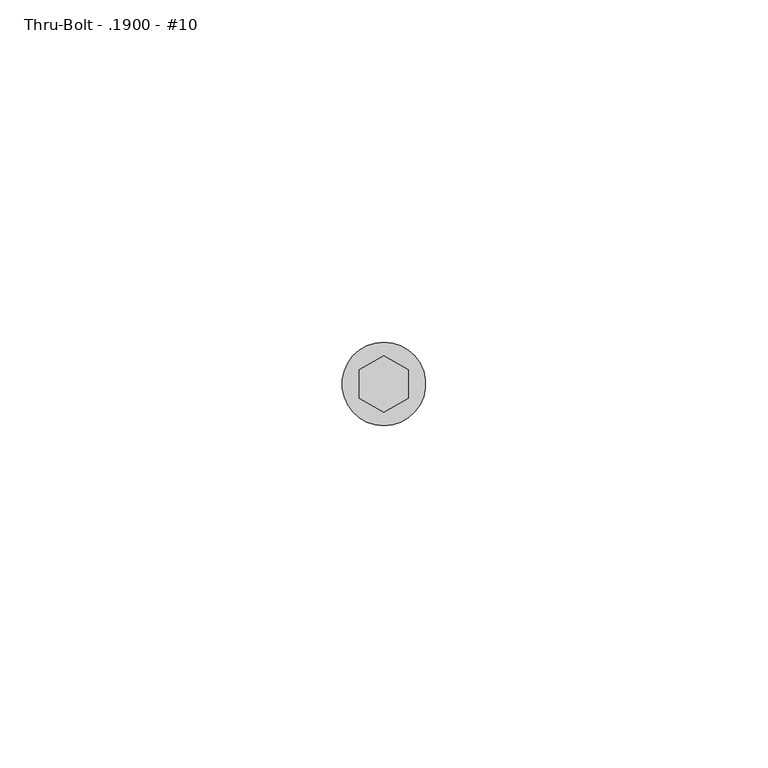
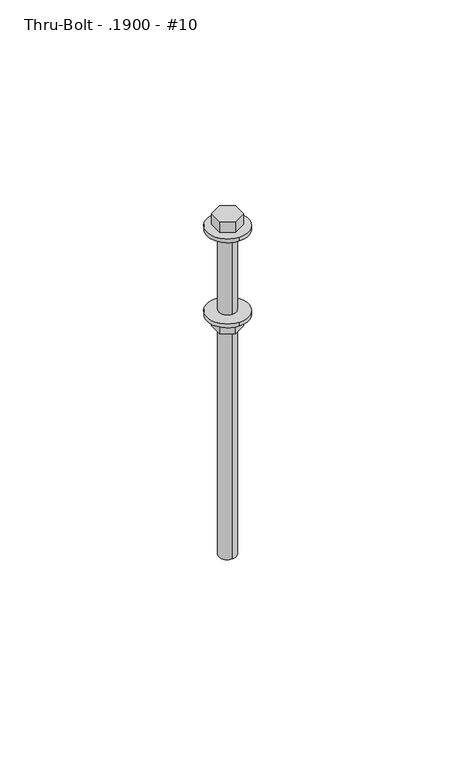
"""IFC4 building model written with IfcOpenShell, lengths in millimetres: fastener geometry, 060523 - W_P_C - Fastenings - Generic : Thru-Bolt - .1900 - #10."""

from ifc_helpers import new_model, si_unit, point, frame, origin, origin_with_axes, origin_2d, place, context, project, spatial, polyline, circle_curve, trimmed, segment, composite_curve, outline, extrude, source, transform, mapped, element, save


def thru_bolt_1900_10_18a4092c(model_context):
    return source(origin(), model_context, "Body", "SweptSolid", [
        extrude(outline(composite_curve([segment(trimmed(circle_curve(origin_2d(), 6.1019531), [point((0.0, 6.1019531))], [point((0.0, -6.1019531))], False, "CARTESIAN"), True, "CONTINUOUS"), segment(trimmed(circle_curve(origin_2d(), 6.1019531), [point((0.0, -6.1019531))], [point((0.0, 6.1019531))], False, "CARTESIAN"), True, "CONTINUOUS")], self_intersect=False)), origin_with_axes(), (0.0, 0.0, 1.0), 1.190625),
        extrude(outline(composite_curve([segment(trimmed(circle_curve(origin_2d(), 6.1019531), [point((0.0, 6.1019531))], [point((0.0, -6.1019531))], False, "CARTESIAN"), True, "CONTINUOUS"), segment(trimmed(circle_curve(origin_2d(), 6.1019531), [point((0.0, -6.1019531))], [point((0.0, 6.1019531))], False, "CARTESIAN"), True, "CONTINUOUS")], self_intersect=False)), frame((0.0, 0.0, -26.590625), z_axis=(0.0, 0.0, 1.0), x_axis=(1.0, 0.0, 0.0)), (0.0, 0.0, 1.0), 1.190625),
        extrude(outline(polyline([(-3.571875, -2.062223), (-3.571875, 2.062223), (0.0, 4.124446), (3.571875, 2.062223), (3.571875, -2.062223), (0.0, -4.124446), (-3.571875, -2.062223)])), frame((0.0, 0.0, -30.1625), z_axis=(0.0, 0.0, 1.0), x_axis=(1.0, 0.0, 0.0)), (0.0, 0.0, 1.0), 3.571875),
        extrude(outline(polyline([(-3.571875, 2.062223), (0.0, 4.124446), (3.571875, 2.062223), (3.571875, -2.062223), (0.0, -4.124446), (-3.571875, -2.062223), (-3.571875, 2.062223)])), frame((0.0, 0.0, 1.190625), z_axis=(0.0, 0.0, 1.0), x_axis=(1.0, 0.0, 0.0)), (0.0, 0.0, 1.0), 3.571875),
        extrude(outline(composite_curve([segment(trimmed(circle_curve(origin_2d(), 2.5300781), [point((0.0, -2.5300781))], [point((0.0, 2.5300781))], False, "CARTESIAN"), True, "CONTINUOUS"), segment(trimmed(circle_curve(origin_2d(), 2.5300781), [point((0.0, 2.5300781))], [point((0.0, -2.5300781))], False, "CARTESIAN"), True, "CONTINUOUS")], self_intersect=False)), frame((0.0, 0.0, -101.6), z_axis=(0.0, 0.0, 1.0), x_axis=(1.0, 0.0, 0.0)), (0.0, 0.0, 1.0), 102.790625),
    ])


if __name__ == "__main__":
    model = new_model("IFC4")
    model_context = context("Model", 3, world=origin())
    ifc_project = project(units=[si_unit("LENGTHUNIT", "METRE", prefix="MILLI")], contexts=[model_context])
    site = spatial("IfcSite", under=ifc_project)
    building = spatial("IfcBuilding", under=site)
    placement = place(None, origin())
    thru_bolt_1900_10_shape = thru_bolt_1900_10_18a4092c(model_context)
    element("IfcFastener", 1, ObjectType="060523 - W_P_C - Fastenings - Generic : Thru-Bolt - .1900 - #10", at=placement, inside=building, context=model_context, shape_type="MappedRepresentation", body=[
        mapped(thru_bolt_1900_10_shape, transform((0.0, 0.0, 0.0), x_axis=(1.0, 0.0, 0.0), y_axis=(0.0, 1.0, 0.0), z_axis=(0.0, 0.0, 1.0))),
    ])
    save(model, "model.ifc")

# Revit data of these elements
# Type "060523 - W_P_C - Fastenings - Generic : Thru-Bolt - .1900 - #10"
#   Washer_Thickness = 0' - 0 3/64"
#   Washer Radius = 0' - 0.24023"
#   Washer Offset - Head = 0' - 0 3/64"
#   Washer Offset = 0' - 0 3/64"
#   Thickness_of_Substrate [instance default] = 0' - 1"
#   Side = 0' - 0.1626"
#   Radius = 0' - 0.09961"
#   Length [instance default] = 0' - 4"
#   Head Size = 0' - 0 9/32"
#   Head Radius = 0' - 0 9/64"
#   Head Height = 0' - 0 9/64"
#   Double Diameter = 0' - 0 51/128"
#   Diameter = 0' - 0 51/256"
#   Default Elevation = 4' - 0"
#   Washer_Nut_Visibility = yes
#   Washer_Head_Visibility = yes
#   Round_Head_Visibility = no
#   Point Visibility = no
#   Nut_Visibility = yes
#   Hex_Head_Visiblilty = yes
#   Washer Material = none
#   Bolt Material (Size) = AT SILL - FASTENER AT 24" O.C.
# Element 1 (IfcFastener, "060523 - W_P_C - Fastenings - Generic : Thru-Bolt - .1900 - #10")
#   Materials on its faces: "AT SILL - FASTENER AT 24\" O.C."
# Materials
#   "AT SILL - FASTENER AT 24\" O.C.": class "Generic", colour RGB 120 120 120, transparency 0, Cost = 0
